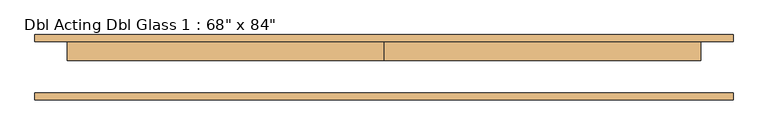
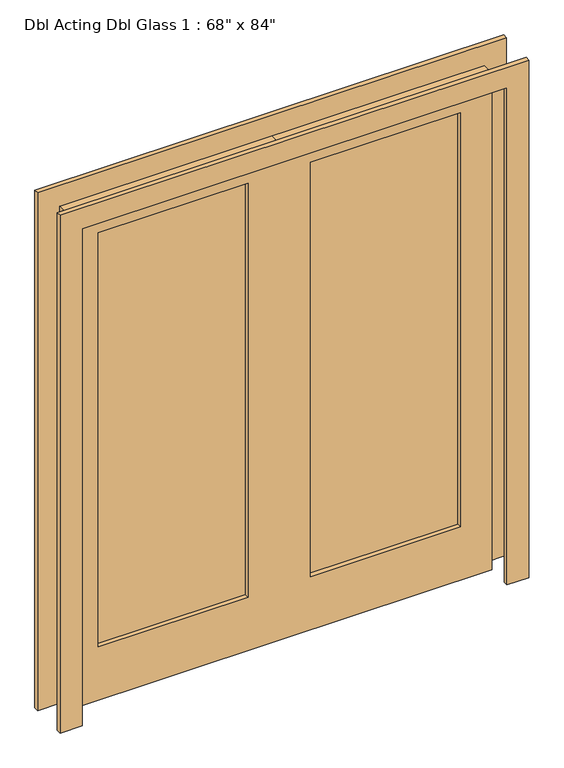
"""IFC4 building model written with IfcOpenShell, lengths in millimetres: door geometry."""

from ifc_helpers import new_model, si_unit, frame, origin, place, context, project, spatial, polyline, outline, extrude, source, transform, mapped, element, save


def door_f1125a27(model_context):
    return source(origin(), model_context, "Body", "SweptSolid", [
        extrude(outline(polyline([(127.0, 76.2), (736.6, 76.2), (736.6, 63.5), (127.0, 63.5), (127.0, 76.2)])), frame((0.0, 0.0, 228.6), z_axis=(0.0, 0.0, 1.0), x_axis=(1.0, 0.0, 0.0)), (0.0, 0.0, 1.0), 1778.0),
        extrude(outline(polyline([(-736.6, 76.2), (-127.0, 76.2), (-127.0, 63.5), (-736.6, 63.5), (-736.6, 76.2)])), frame((0.0, 0.0, 228.6), z_axis=(0.0, 0.0, 1.0), x_axis=(1.0, 0.0, 0.0)), (0.0, 0.0, 1.0), 1778.0),
        extrude(outline(polyline([(2133.6, 0.0), (2133.6, -863.6), (0.0, -863.6), (0.0, 0.0), (0.0, 863.6), (2133.6, 863.6), (2133.6, 0.0)]), holes=[polyline([(2006.6, 127.0), (2006.6, 736.6), (228.6, 736.6), (228.6, 127.0), (2006.6, 127.0)]), polyline([(2006.6, -127.0), (228.6, -127.0), (228.6, -736.6), (2006.6, -736.6), (2006.6, -127.0)])]), frame((0.0, 44.45, 0.0), z_axis=(0.0, 1.0, 0.0), x_axis=(0.0, 0.0, 1.0)), (0.0, 0.0, 1.0), 50.8),
        extrude(outline(polyline([(2133.6, -863.6), (2133.6, 863.6), (0.0, 863.6), (0.0, 952.5), (2222.5, 952.5), (2222.5, -952.5), (0.0, -952.5), (0.0, -863.6), (2133.6, -863.6)])), frame((0.0, -63.5, 0.0), z_axis=(0.0, 1.0, 0.0), x_axis=(0.0, 0.0, 1.0)), (0.0, 0.0, 1.0), 19.05),
        extrude(outline(polyline([(2133.6, -863.6), (2133.6, 863.6), (0.0, 863.6), (0.0, 952.5), (2222.5, 952.5), (2222.5, -952.5), (0.0, -952.5), (0.0, -863.6), (2133.6, -863.6)])), frame((0.0, 95.25, 0.0), z_axis=(0.0, 1.0, 0.0), x_axis=(0.0, 0.0, 1.0)), (0.0, 0.0, 1.0), 19.05),
    ])


if __name__ == "__main__":
    model = new_model("IFC4")
    model_context = context("Model", 3, world=origin())
    ifc_project = project(units=[si_unit("LENGTHUNIT", "METRE", prefix="MILLI")], contexts=[model_context])
    site = spatial("IfcSite", under=ifc_project)
    building = spatial("IfcBuilding", under=site)
    placement = place(None, origin())
    door_shape = door_f1125a27(model_context)
    element("IfcDoor", 1, ObjectType="Dbl Acting Dbl Glass 1 : 68\" x 84\"", at=placement, inside=building, context=model_context, shape_type="MappedRepresentation", body=[
        mapped(door_shape, transform((0.0, 0.0, 0.0), x_axis=(1.0, 0.0, 0.0), y_axis=(0.0, 1.0, 0.0), z_axis=(0.0, 0.0, 1.0))),
    ])
    save(model, "model.ifc")

# Revit data of these elements
# Type "Dbl Acting Dbl Glass 1 : 68\" x 84\""
#   Type Mark = "33"
#   Door Thickness = 0' - 2"
#   Height = 7' - 0"
#   Rail Width - Base = 0' - 9"
#   Rail Width - Head = 0' - 5"
#   Stile Width - Hinge = 0' - 5"
#   Stile Width - Lock = 0' - 5"
#   Trim Projection Ext. = 0' - 0 3/4"
#   Trim Projection Int. = 0' - 0 3/4"
#   Trim Width Ext. = 0' - 3 1/2"
#   Trim Width Int. = 0' - 3 1/2"
#   Width = 5' - 8"
#   Function = 0
#   Wall Closure = (empty or 0)
# Element 1 (IfcDoor, "Dbl Acting Dbl Glass 1 : 68\" x 84\"")
#   Materials on its faces: "Glass"
# Materials
#   "Glass": class "Glass", colour RGB 0 128 192, transparency 0.75, Description = "Soda Lime Glass", Cost = 0
